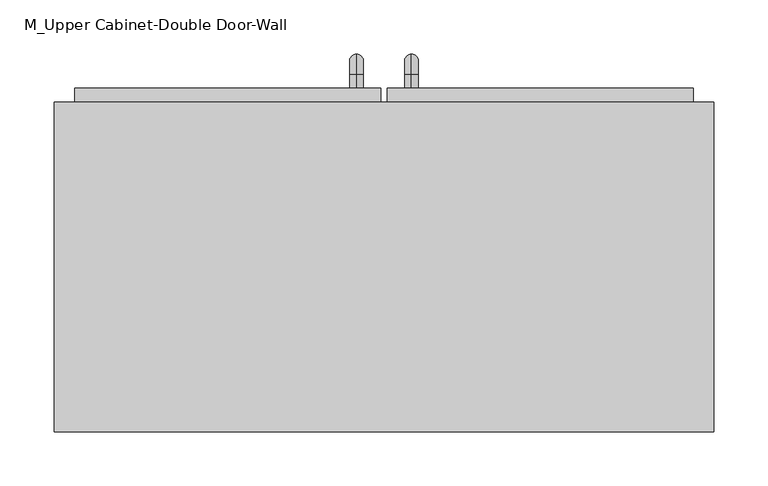
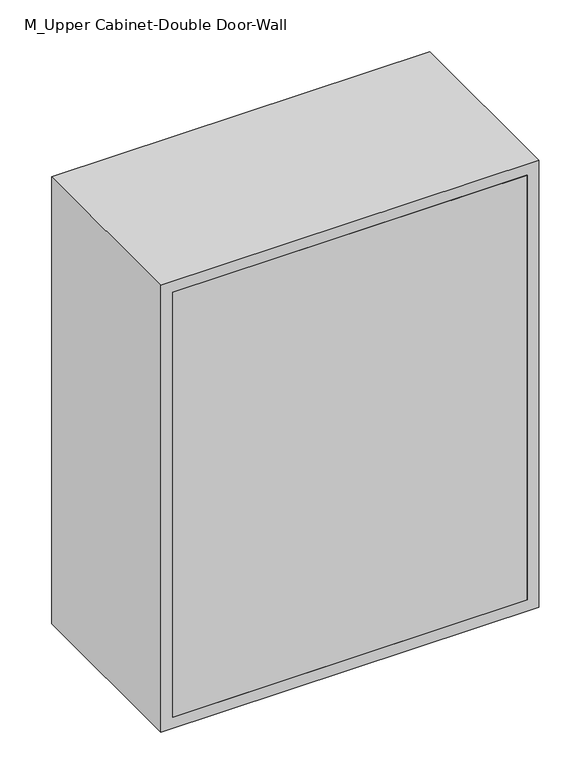
"""IFC4 building model written with IfcOpenShell, lengths in millimetres: furniture geometry, M_Upper Cabinet-Double Door-Wall : 24W X 30H."""

from ifc_helpers import new_model, si_unit, point, frame, origin, place, context, project, spatial, polyline, circle_curve, ellipse_curve, trimmed, outline, extrude, source, transform, mapped, element, save
from ifc_brep_helpers import plane_surface, cylinder_surface, revolved_surface, advanced_brep


def m_upper_cabinet_double_door_wall_78e0ec07(model_context):
    return source(origin(), model_context, "Body", "SolidModel", [
        advanced_brep(
        [(55.1711628, 393.7, 1212.85), (55.1711628, 393.7, 1225.55), (55.1711628, 406.4, 1212.85), (55.1711628, 406.4, 1225.55), (55.1711628, 425.45, 1206.5), (55.1711628, 412.75, 1206.5), (55.1711628, 412.75, 1130.3), (55.1711628, 425.45, 1130.3), (55.1711628, 406.4, 1111.25), (55.1711628, 406.4, 1123.95), (55.1711628, 393.7, 1123.95), (55.1711628, 393.7, 1111.25)],
        [
            (0, 1, circle_curve(frame((55.1711628, 393.7, 1219.2), z_axis=(0.0, -1.0, 0.0), x_axis=(0.0, 0.0, -1.0)), 6.35)),
            (1, 0, circle_curve(frame((55.1711628, 393.7, 1219.2), z_axis=(0.0, -1.0, 0.0), x_axis=(0.0, 0.0, -1.0)), 6.35)),
            (0, 2),
            (2, 3, circle_curve(frame((55.1711628, 406.4, 1219.2), z_axis=(0.0, -1.0, 0.0), x_axis=(0.0, 0.0, -1.0)), 6.35)),
            (3, 1),
            (3, 2, circle_curve(frame((55.1711628, 406.4, 1219.2), z_axis=(0.0, -1.0, 0.0), x_axis=(0.0, 0.0, -1.0)), 6.35)),
            (4, 3, circle_curve(frame((55.1711628, 406.4, 1206.5), z_axis=(1.0, 0.0, 0.0), x_axis=(0.0, 0.0, 1.0)), 19.05)),
            (2, 5, circle_curve(frame((55.1711628, 406.4, 1206.5), z_axis=(-1.0, 0.0, 0.0), x_axis=(0.0, 0.0, 1.0)), 6.35)),
            (5, 4, circle_curve(frame((55.1711628, 419.1, 1206.5), z_axis=(0.0, 0.0, 1.0), x_axis=(0.0, -1.0, 0.0)), 6.35)),
            (4, 5, circle_curve(frame((55.1711628, 419.1, 1206.5), z_axis=(0.0, 0.0, 1.0), x_axis=(0.0, -1.0, 0.0)), 6.35)),
            (5, 6),
            (6, 7, circle_curve(frame((55.1711628, 419.1, 1130.3), z_axis=(0.0, 0.0, 1.0), x_axis=(0.0, -1.0, 0.0)), 6.35)),
            (7, 4),
            (7, 6, circle_curve(frame((55.1711628, 419.1, 1130.3), z_axis=(0.0, 0.0, 1.0), x_axis=(0.0, -1.0, 0.0)), 6.35)),
            (8, 7, circle_curve(frame((55.1711628, 406.4, 1130.3), z_axis=(1.0, 0.0, 0.0), x_axis=(0.0, 1.0, 0.0)), 19.05)),
            (6, 9, circle_curve(frame((55.1711628, 406.4, 1130.3), z_axis=(-1.0, 0.0, 0.0), x_axis=(0.0, 1.0, 0.0)), 6.35)),
            (9, 8, circle_curve(frame((55.1711628, 406.4, 1117.6), z_axis=(0.0, 1.0, 0.0), x_axis=(0.0, 0.0, 1.0)), 6.35)),
            (8, 9, circle_curve(frame((55.1711628, 406.4, 1117.6), z_axis=(0.0, 1.0, 0.0), x_axis=(0.0, 0.0, 1.0)), 6.35)),
            (10, 11, circle_curve(frame((55.1711628, 393.7, 1117.6), z_axis=(0.0, -1.0, 0.0), x_axis=(0.0, 0.0, 1.0)), 6.35)),
            (11, 10, circle_curve(frame((55.1711628, 393.7, 1117.6), z_axis=(0.0, -1.0, 0.0), x_axis=(0.0, 0.0, 1.0)), 6.35)),
            (9, 10),
            (11, 8),
        ],
        [
            plane_surface(frame((48.8211628, 393.7, 1219.2), z_axis=(0.0, -1.0, 0.0), x_axis=(0.0, 0.0, 1.0))),
            cylinder_surface(frame((55.1711628, 393.7, 1219.2), z_axis=(0.0, -1.0, 0.0), x_axis=(0.0, 0.0, -1.0)), 6.35),
            revolved_surface(trimmed(ellipse_curve(frame((55.1711628, 406.4, 1219.2), z_axis=(0.0, -1.0, 0.0), x_axis=(0.0, 0.0, -1.0)), 6.35, 6.35), [point((55.1711628, 406.4, 1212.85))], [point((55.1711628, 406.4, 1225.55))], True, "CARTESIAN"), (55.1711628, 406.4, 1206.5), (-1.0, 0.0, 0.0)),
            revolved_surface(trimmed(ellipse_curve(frame((55.1711628, 406.4, 1219.2), z_axis=(0.0, -1.0, 0.0), x_axis=(0.0, 0.0, -1.0)), 6.35, 6.35), [point((55.1711628, 406.4, 1225.55))], [point((55.1711628, 406.4, 1212.85))], True, "CARTESIAN"), (55.1711628, 406.4, 1206.5), (-1.0, 0.0, 0.0)),
            cylinder_surface(frame((55.1711628, 419.1, 1206.5), z_axis=(0.0, 0.0, 1.0), x_axis=(0.0, -1.0, 0.0)), 6.35),
            revolved_surface(trimmed(ellipse_curve(frame((55.1711628, 419.1, 1130.3), z_axis=(0.0, 0.0, 1.0), x_axis=(0.0, -1.0, 0.0)), 6.35, 6.35), [point((55.1711628, 412.75, 1130.3))], [point((55.1711628, 425.45, 1130.3))], True, "CARTESIAN"), (55.1711628, 406.4, 1130.3), (-1.0, 0.0, 0.0)),
            revolved_surface(trimmed(ellipse_curve(frame((55.1711628, 419.1, 1130.3), z_axis=(0.0, 0.0, 1.0), x_axis=(0.0, -1.0, 0.0)), 6.35, 6.35), [point((55.1711628, 425.45, 1130.3))], [point((55.1711628, 412.75, 1130.3))], True, "CARTESIAN"), (55.1711628, 406.4, 1130.3), (-1.0, 0.0, 0.0)),
            plane_surface(frame((48.8211628, 393.7, 1117.6), z_axis=(0.0, -1.0, 0.0), x_axis=(0.0, 0.0, -1.0))),
            cylinder_surface(frame((55.1711628, 406.4, 1117.6), z_axis=(0.0, 1.0, 0.0), x_axis=(0.0, 0.0, 1.0)), 6.35),
        ],
        [
            (0, [[1, 2]]),
            (1, [[-1, 3, 4, 5]]),
            (1, [[-2, -5, 6, -3]]),
            (2, [[7, -4, 8, 9]]),
            (3, [[-8, -6, -7, 10]]),
            (4, [[-9, 11, 12, 13]]),
            (4, [[-10, -13, 14, -11]]),
            (5, [[15, -12, 16, 17]]),
            (6, [[-16, -14, -15, 18]]),
            (7, [[19, 20]]),
            (8, [[-17, 21, -20, 22]]),
            (8, [[-18, -22, -19, -21]]),
        ],
    ),
        advanced_brep(
        [(4.3711628, 393.7, 1212.85), (4.3711628, 393.7, 1225.55), (4.3711628, 406.4, 1212.85), (4.3711628, 406.4, 1225.55), (4.3711628, 425.45, 1206.5), (4.3711628, 412.75, 1206.5), (4.3711628, 412.75, 1130.3), (4.3711628, 425.45, 1130.3), (4.3711628, 406.4, 1111.25), (4.3711628, 406.4, 1123.95), (4.3711628, 393.7, 1123.95), (4.3711628, 393.7, 1111.25)],
        [
            (0, 1, circle_curve(frame((4.3711628, 393.7, 1219.2), z_axis=(0.0, -1.0, 0.0), x_axis=(0.0, 0.0, 1.0)), 6.35)),
            (1, 0, circle_curve(frame((4.3711628, 393.7, 1219.2), z_axis=(0.0, -1.0, 0.0), x_axis=(0.0, 0.0, 1.0)), 6.35)),
            (0, 2),
            (2, 3, circle_curve(frame((4.3711628, 406.4, 1219.2), z_axis=(0.0, -1.0, 0.0), x_axis=(0.0, 0.0, 1.0)), 6.35)),
            (3, 1),
            (3, 2, circle_curve(frame((4.3711628, 406.4, 1219.2), z_axis=(0.0, -1.0, 0.0), x_axis=(0.0, 0.0, 1.0)), 6.35)),
            (4, 3, circle_curve(frame((4.3711628, 406.4, 1206.5), z_axis=(1.0, 0.0, 0.0), x_axis=(0.0, 0.0, 1.0)), 19.05)),
            (2, 5, circle_curve(frame((4.3711628, 406.4, 1206.5), z_axis=(-1.0, 0.0, 0.0), x_axis=(0.0, 0.0, 1.0)), 6.35)),
            (5, 4, circle_curve(frame((4.3711628, 419.1, 1206.5), z_axis=(0.0, 0.0, 1.0), x_axis=(0.0, 1.0, 0.0)), 6.35)),
            (4, 5, circle_curve(frame((4.3711628, 419.1, 1206.5), z_axis=(0.0, 0.0, 1.0), x_axis=(0.0, 1.0, 0.0)), 6.35)),
            (5, 6),
            (6, 7, circle_curve(frame((4.3711628, 419.1, 1130.3), z_axis=(0.0, 0.0, 1.0), x_axis=(0.0, 1.0, 0.0)), 6.35)),
            (7, 4),
            (7, 6, circle_curve(frame((4.3711628, 419.1, 1130.3), z_axis=(0.0, 0.0, 1.0), x_axis=(0.0, 1.0, 0.0)), 6.35)),
            (8, 7, circle_curve(frame((4.3711628, 406.4, 1130.3), z_axis=(1.0, 0.0, 0.0), x_axis=(0.0, 1.0, 0.0)), 19.05)),
            (6, 9, circle_curve(frame((4.3711628, 406.4, 1130.3), z_axis=(-1.0, 0.0, 0.0), x_axis=(0.0, 1.0, 0.0)), 6.35)),
            (9, 8, circle_curve(frame((4.3711628, 406.4, 1117.6), z_axis=(0.0, 1.0, 0.0), x_axis=(0.0, 0.0, -1.0)), 6.35)),
            (8, 9, circle_curve(frame((4.3711628, 406.4, 1117.6), z_axis=(0.0, 1.0, 0.0), x_axis=(0.0, 0.0, -1.0)), 6.35)),
            (10, 11, circle_curve(frame((4.3711628, 393.7, 1117.6), z_axis=(0.0, -1.0, 0.0), x_axis=(0.0, 0.0, -1.0)), 6.35)),
            (11, 10, circle_curve(frame((4.3711628, 393.7, 1117.6), z_axis=(0.0, -1.0, 0.0), x_axis=(0.0, 0.0, -1.0)), 6.35)),
            (9, 10),
            (11, 8),
        ],
        [
            plane_surface(frame((-1.9788372, 393.7, 1219.2), z_axis=(0.0, -1.0, 0.0), x_axis=(0.0, 0.0, 1.0))),
            cylinder_surface(frame((4.3711628, 393.7, 1219.2), z_axis=(0.0, -1.0, 0.0), x_axis=(0.0, 0.0, 1.0)), 6.35),
            revolved_surface(trimmed(ellipse_curve(frame((4.3711628, 406.4, 1219.2), z_axis=(0.0, -1.0, 0.0), x_axis=(0.0, 0.0, 1.0)), 6.35, 6.35), [point((4.3711628, 406.4, 1212.85))], [point((4.3711628, 406.4, 1225.55))], True, "CARTESIAN"), (4.3711628, 406.4, 1206.5), (-1.0, 0.0, 0.0)),
            revolved_surface(trimmed(ellipse_curve(frame((4.3711628, 406.4, 1219.2), z_axis=(0.0, -1.0, 0.0), x_axis=(0.0, 0.0, 1.0)), 6.35, 6.35), [point((4.3711628, 406.4, 1225.55))], [point((4.3711628, 406.4, 1212.85))], True, "CARTESIAN"), (4.3711628, 406.4, 1206.5), (-1.0, 0.0, 0.0)),
            cylinder_surface(frame((4.3711628, 419.1, 1206.5), z_axis=(0.0, 0.0, 1.0), x_axis=(0.0, 1.0, 0.0)), 6.35),
            revolved_surface(trimmed(ellipse_curve(frame((4.3711628, 419.1, 1130.3), z_axis=(0.0, 0.0, 1.0), x_axis=(0.0, 1.0, 0.0)), 6.35, 6.35), [point((4.3711628, 412.75, 1130.3))], [point((4.3711628, 425.45, 1130.3))], True, "CARTESIAN"), (4.3711628, 406.4, 1130.3), (-1.0, 0.0, 0.0)),
            revolved_surface(trimmed(ellipse_curve(frame((4.3711628, 419.1, 1130.3), z_axis=(0.0, 0.0, 1.0), x_axis=(0.0, 1.0, 0.0)), 6.35, 6.35), [point((4.3711628, 425.45, 1130.3))], [point((4.3711628, 412.75, 1130.3))], True, "CARTESIAN"), (4.3711628, 406.4, 1130.3), (-1.0, 0.0, 0.0)),
            plane_surface(frame((-1.9788372, 393.7, 1117.6), z_axis=(0.0, -1.0, 0.0), x_axis=(0.0, 0.0, -1.0))),
            cylinder_surface(frame((4.3711628, 406.4, 1117.6), z_axis=(0.0, 1.0, 0.0), x_axis=(0.0, 0.0, -1.0)), 6.35),
        ],
        [
            (0, [[1, 2]]),
            (1, [[-1, 3, 4, 5]]),
            (1, [[-2, -5, 6, -3]]),
            (2, [[7, -4, 8, 9]]),
            (3, [[-8, -6, -7, 10]]),
            (4, [[-9, 11, 12, 13]]),
            (4, [[-10, -13, 14, -11]]),
            (5, [[15, -12, 16, 17]]),
            (6, [[-16, -14, -15, 18]]),
            (7, [[19, 20]]),
            (8, [[-17, 21, -20, 22]]),
            (8, [[-18, -22, -19, -21]]),
        ],
    ),
        extrude(outline(polyline([(32.9461628, 393.7), (315.5211628, 393.7), (315.5211628, 361.95), (32.9461628, 361.95), (32.9461628, 393.7)])), frame((0.0, 0.0, 1085.85), z_axis=(0.0, 0.0, 1.0), x_axis=(1.0, 0.0, 0.0)), (0.0, 0.0, 1.0), 723.9),
        extrude(outline(polyline([(-255.9788372, 393.7), (26.5961628, 393.7), (26.5961628, 361.95), (-255.9788372, 361.95), (-255.9788372, 393.7)])), frame((0.0, 0.0, 1085.85), z_axis=(0.0, 0.0, 1.0), x_axis=(1.0, 0.0, 0.0)), (0.0, 0.0, 1.0), 723.9),
        extrude(outline(polyline([(315.5211628, 76.2), (-255.9788372, 76.2), (-255.9788372, 95.25), (315.5211628, 95.25), (315.5211628, 76.2)])), frame((0.0, 0.0, 1085.85), z_axis=(0.0, 0.0, 1.0), x_axis=(1.0, 0.0, 0.0)), (0.0, 0.0, 1.0), 723.9),
        extrude(outline(polyline([(1828.8, -275.0288372), (1066.8, -275.0288372), (1066.8, 334.5711628), (1828.8, 334.5711628), (1828.8, -275.0288372)]), holes=[polyline([(1809.75, -255.9788372), (1809.75, 315.5211628), (1085.85, 315.5211628), (1085.85, -255.9788372), (1809.75, -255.9788372)])]), frame((0.0, 76.2, 0.0), z_axis=(0.0, 1.0, 0.0), x_axis=(0.0, 0.0, 1.0)), (0.0, 0.0, 1.0), 304.8),
    ])


if __name__ == "__main__":
    model = new_model("IFC4")
    model_context = context("Model", 3, world=origin())
    ifc_project = project(units=[si_unit("LENGTHUNIT", "METRE", prefix="MILLI")], contexts=[model_context])
    site = spatial("IfcSite", under=ifc_project)
    building = spatial("IfcBuilding", under=site)
    placement = place(None, origin())
    m_upper_cabinet_double_door_wall_shape = m_upper_cabinet_double_door_wall_78e0ec07(model_context)
    element("IfcFurniture", 1, ObjectType="M_Upper Cabinet-Double Door-Wall : 24W X 30H", at=placement, inside=building, context=model_context, shape_type="MappedRepresentation", body=[
        mapped(m_upper_cabinet_double_door_wall_shape, transform((0.0, 0.0, 0.0), x_axis=(1.0, 0.0, 0.0), y_axis=(0.0, 1.0, 0.0), z_axis=(0.0, 0.0, 1.0))),
    ])
    save(model, "model.ifc")

# Revit data of these elements
# Type "M_Upper Cabinet-Double Door-Wall : 24W X 30H"
#   Depth = 1' - 0"
#   Height = 2' - 6"
#   Top Of Cabinet = 6' - 0"
#   Width = 2' - 0"
#   Cabinet Material = none
#   Door/Drawer Material = none
#   Handle Material = Cabinets - Handles
# Element 1 (IfcFurniture, "M_Upper Cabinet-Double Door-Wall : 24W X 30H")
#   Materials on its faces: "MAX HEIGHT OF  COUNTERTOP 34\"", "Cabinets - Handles"
# Materials
#   "Cabinets - Handles": class "Metal", colour RGB 57 57 57, transparency 0
#   "MAX HEIGHT OF  COUNTERTOP 34\"": class "Generic", colour RGB 181 181 181, transparency 0, Cost = 0
